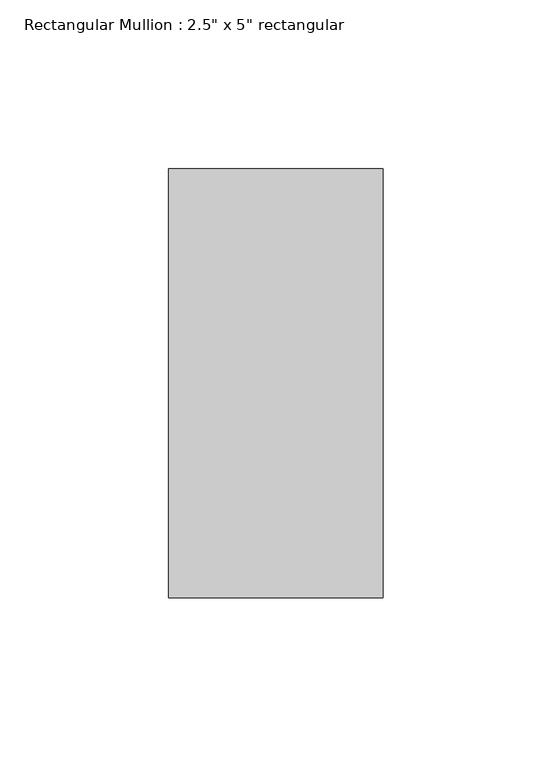
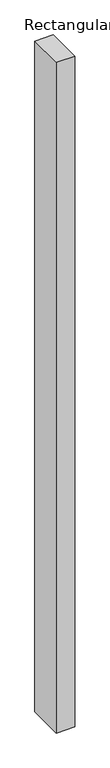
"""IFC4 building model written with IfcOpenShell, lengths in millimetres: member geometry."""

import ifcopenshell
import ifcopenshell.guid

model = None  # the IFC model being written
_history = None  # IfcOwnerHistory: only IFC2X3 demands one
_inside = {}  # id of a spatial element -> (the spatial element, [elements in it])
_under = {}  # id of a project, library or spatial element -> (it, [spatial elements below it])
_declared = {}  # id of a project -> (the project, [libraries it declares])
_typed = {}  # id of a type object -> (the type object, [elements of that type])
_made_of = {}  # id of a material, layer set ... -> (it, [elements and type objects made of it])


def new_model(schema):
    """Start an empty IFC model of exactly this schema.

    Asked for "IFC4X3", IfcOpenShell would pick the latest addendum, in which some entities
    have other attributes; the version numbers below select the first issue.
    IFC2X3 requires an IfcOwnerHistory on every rooted entity: one is made here for all.
    """
    global model, _history
    if schema == "IFC4X3":
        model = ifcopenshell.file(schema_version=(4, 3, 0, 0))
    else:
        model = ifcopenshell.file(schema=schema)
    _inside.clear()
    _under.clear()
    _declared.clear()
    _typed.clear()
    _made_of.clear()
    _history = None
    if model.schema == "IFC2X3":
        org = make("IfcOrganization", Name="unknown")
        user = make(
            "IfcPersonAndOrganization",
            ThePerson=make("IfcPerson", FamilyName="unknown"),
            TheOrganization=org,
        )
        app = make(
            "IfcApplication",
            ApplicationDeveloper=org,
            Version="unknown",
            ApplicationFullName="unknown",
            ApplicationIdentifier="unknown",
        )
        _history = make(
            "IfcOwnerHistory",
            OwningUser=user,
            OwningApplication=app,
            ChangeAction="ADDED",
            CreationDate=0,
        )
    return model


def make(cls, **values):
    """One entity of the class cls with the attributes given. An attribute that is None is left unset."""
    return model.create_entity(
        cls, **{name: value for name, value in values.items() if value is not None}
    )


def rooted(cls, **values):
    """An entity with a GlobalId (a new one), such as an element, a storey or a relation."""
    return make(cls, GlobalId=ifcopenshell.guid.new(), OwnerHistory=_history, **values)


def si_unit(unit_type, name, prefix=None):
    """IfcSIUnit, for example si_unit("LENGTHUNIT", "METRE", prefix="MILLI")."""
    return make("IfcSIUnit", UnitType=unit_type, Prefix=prefix, Name=name)


def assignment(units):
    """IfcUnitAssignment: the units of a project."""
    return None if units is None else make("IfcUnitAssignment", Units=units)


def point(xyz):
    """IfcCartesianPoint."""
    return None if xyz is None else make("IfcCartesianPoint", Coordinates=xyz)


def direction(xyz):
    """IfcDirection."""
    return None if xyz is None else make("IfcDirection", DirectionRatios=xyz)


def frame(location, z_axis=None, x_axis=None):
    """IfcAxis2Placement3D, a coordinate frame: its origin and axes. An axis left out is left unset."""
    return make(
        "IfcAxis2Placement3D",
        Location=point(location),
        Axis=direction(z_axis),
        RefDirection=direction(x_axis),
    )


def origin():
    """The frame at (0, 0, 0) with its axes left unset."""
    return frame((0.0, 0.0, 0.0))


def place(relative_to, where):
    """IfcLocalPlacement: puts the frame where relative to a parent placement (None: the world)."""
    return make(
        "IfcLocalPlacement", PlacementRelTo=relative_to, RelativePlacement=where
    )


def context(
    kind, dimensions, precision=None, world=None, true_north=None, identifier=None
):
    """IfcGeometricRepresentationContext, for example the 3D "Model" context."""
    return make(
        "IfcGeometricRepresentationContext",
        ContextIdentifier=identifier,
        ContextType=kind,
        CoordinateSpaceDimension=dimensions,
        Precision=precision,
        WorldCoordinateSystem=world,
        TrueNorth=true_north,
    )


def project(units=None, contexts=None):
    """IfcProject with its units and contexts."""
    return rooted(
        "IfcProject",
        Name="project",
        RepresentationContexts=contexts,
        UnitsInContext=assignment(units),
    )


def spatial(cls, under=None, at=None, **own):
    """A site, building, storey or space (cls), placed at a placement, below another one or the project."""
    s = rooted(cls, ObjectPlacement=at, **own)
    if under is not None:
        _under.setdefault(under.id(), (under, []))[1].append(s)
    return s


def polyline(points):
    """IfcPolyline through the points."""
    return make("IfcPolyline", Points=[point(p) for p in points])


def outline(outer, holes=None, kind="AREA"):
    """IfcArbitraryClosedProfileDef: a profile drawn as a closed curve; with holes, ...WithVoids."""
    if holes is None:
        return make("IfcArbitraryClosedProfileDef", ProfileType=kind, OuterCurve=outer)
    return make(
        "IfcArbitraryProfileDefWithVoids",
        ProfileType=kind,
        OuterCurve=outer,
        InnerCurves=holes,
    )


def extrude(swept, where, along, depth):
    """IfcExtrudedAreaSolid: the profile swept, set in the frame where, extruded along a direction by depth."""
    return make(
        "IfcExtrudedAreaSolid",
        SweptArea=swept,
        Position=where,
        ExtrudedDirection=direction(along),
        Depth=depth,
    )


def shape(context_of_items, identifier, shape_type, items):
    """IfcShapeRepresentation: the items that make up one representation, for example the "Body"."""
    return make(
        "IfcShapeRepresentation",
        ContextOfItems=context_of_items,
        RepresentationIdentifier=identifier,
        RepresentationType=shape_type,
        Items=items,
    )


def source(mapping_origin, context_of_items, identifier, shape_type, items):
    """IfcRepresentationMap: a shape defined once, which mapped items show again and again."""
    return make(
        "IfcRepresentationMap",
        MappingOrigin=mapping_origin,
        MappedRepresentation=shape(context_of_items, identifier, shape_type, items),
    )


def transform(
    local_origin,
    x_axis=None,
    y_axis=None,
    z_axis=None,
    scale=None,
    scale2=None,
    scale3=None,
    uniform=True,
):
    """IfcCartesianTransformationOperator3D, or its non-uniform kind. x_axis, y_axis, z_axis: its Axis1, 2, 3."""
    if uniform:
        return make(
            "IfcCartesianTransformationOperator3D",
            Axis1=direction(x_axis),
            Axis2=direction(y_axis),
            LocalOrigin=point(local_origin),
            Scale=scale,
            Axis3=direction(z_axis),
        )
    return make(
        "IfcCartesianTransformationOperator3DnonUniform",
        Axis1=direction(x_axis),
        Axis2=direction(y_axis),
        LocalOrigin=point(local_origin),
        Scale=scale,
        Axis3=direction(z_axis),
        Scale2=scale2,
        Scale3=scale3,
    )


def mapped(mapping_source, mapping_target):
    """IfcMappedItem: shows the shape of a source again, moved by a transform."""
    return make(
        "IfcMappedItem", MappingSource=mapping_source, MappingTarget=mapping_target
    )


def made_of(thing, what):
    """Note that an element or type object is made of a material, layer set ...; save() writes the relation."""
    if what is not None:
        _made_of.setdefault(what.id(), (what, []))[1].append(thing)
    return thing


def element(
    cls,
    number,
    at=None,
    inside=None,
    cuts=None,
    type_object=None,
    material=None,
    context=None,
    identifier="Body",
    shape_type=None,
    held_by="IfcProductDefinitionShape",
    body=None,
    shapes=None,
    **own,
):
    """One element of the class cls, such as IfcWall. Its Tag is "e" and its number.

    at: its placement. inside: the storey or other place that contains it. cuts: it is an
    opening in that element (IfcRelVoidsElement). A single representation is given by context,
    identifier, shape_type and body (its items); several are given by shapes. held_by: the class
    of the entity that holds the representations. save() writes the other relations.
    """
    e = rooted(cls, Tag="e%d" % number, ObjectPlacement=at, **own)
    if body is not None:
        shapes = [shape(context, identifier, shape_type, body)]
    if shapes is not None:
        e.Representation = make(held_by, Representations=shapes)
    if inside is not None:
        _inside.setdefault(inside.id(), (inside, []))[1].append(e)
    if cuts is not None:
        rooted(
            "IfcRelVoidsElement", RelatingBuildingElement=cuts, RelatedOpeningElement=e
        )
    if type_object is not None:
        _typed.setdefault(type_object.id(), (type_object, []))[1].append(e)
    return made_of(e, material)


def aggregate(whole, parts):
    """IfcRelAggregates: a whole, such as a stair, and the parts it consists of."""
    return rooted("IfcRelAggregates", RelatingObject=whole, RelatedObjects=parts)


def save(model, path):
    """Write the relations noted so far, then the file.

    IfcRelAggregates (storeys below a building ...), IfcRelContainedInSpatialStructure (elements
    in a storey), IfcRelDefinesByType, IfcRelAssociatesMaterial and IfcRelDeclares: one each for
    every whole, place, type object, material and project.
    """
    for whole, parts in _under.values():
        aggregate(whole, parts)
    for where, things in _inside.values():
        rooted(
            "IfcRelContainedInSpatialStructure",
            RelatedElements=things,
            RelatingStructure=where,
        )
    for kind, things in _typed.values():
        rooted("IfcRelDefinesByType", RelatedObjects=things, RelatingType=kind)
    for what, things in _made_of.values():
        rooted("IfcRelAssociatesMaterial", RelatedObjects=things, RelatingMaterial=what)
    for by, libraries in _declared.values():
        rooted("IfcRelDeclares", RelatingContext=by, RelatedDefinitions=libraries)
    model.write(path)


def member_f0fea5a5(model_context):
    return source(origin(), model_context, "Body", "SweptSolid", [
        extrude(outline(polyline([(31.75, 63.5), (31.75, -63.5), (-31.75, -63.5), (-31.75, 63.5), (31.75, 63.5)])), frame((0.0, 0.0, -2438.4), z_axis=(0.0, 0.0, 1.0), x_axis=(1.0, 0.0, 0.0)), (0.0, 0.0, 1.0), 2438.4),
    ])


if __name__ == "__main__":
    model = new_model("IFC4")
    model_context = context("Model", 3, world=origin())
    ifc_project = project(units=[si_unit("LENGTHUNIT", "METRE", prefix="MILLI")], contexts=[model_context])
    site = spatial("IfcSite", under=ifc_project)
    building = spatial("IfcBuilding", under=site)
    placement = place(None, origin())
    member_shape = member_f0fea5a5(model_context)
    element("IfcMember", 1, ObjectType="Rectangular Mullion : 2.5\" x 5\" rectangular", at=placement, inside=building, context=model_context, shape_type="MappedRepresentation", body=[
        mapped(member_shape, transform((0.0, 0.0, 0.0), x_axis=(1.0, 0.0, 0.0), y_axis=(0.0, 1.0, 0.0), z_axis=(0.0, 0.0, 1.0))),
    ])
    save(model, "model.ifc")

# Revit data of these elements
# Type "Rectangular Mullion : 2.5\" x 5\" rectangular"
#   built-in parameter 1007304 = 0.416667 (stored number, unit not read)
#   built-in parameter 1007301 = 0.104167 (stored number, unit not read)
#   built-in parameter 1007300 = 0.104167 (stored number, unit not read)
# Element 1 (IfcMember, "Rectangular Mullion : 2.5\" x 5\" rectangular")
#   Materials on its faces: "Metal - Aluminum"
# Materials
#   "Metal - Aluminum": class "Metal", colour RGB 140 140 140, transparency 0
